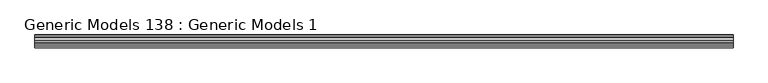
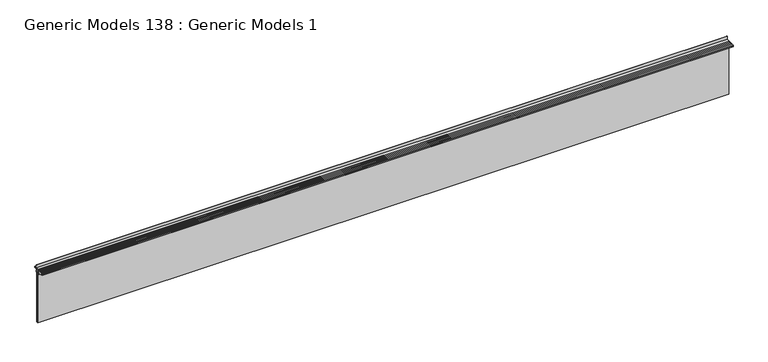
"""IFC4 building model written with IfcOpenShell, lengths in millimetres: proxy geometry, Generic Models 138 : Generic Models 1."""

from ifc_helpers import new_model, si_unit, point, frame, frame_2d, origin, place, context, project, spatial, polyline, circle_curve, trimmed, segment, composite_curve, outline, extrude, source, transform, mapped, element, save


def generic_models_138_generic_models_1_f7e5df14(model_context):
    return source(origin(), model_context, "Body", "SweptSolid", [
        extrude(outline(composite_curve([segment(polyline([(11384.4166338, 129382.901), (11402.4851772, 129382.901), (11402.4851772, 129379.726), (11404.7711811, 129379.726), (11404.7711811, 129382.901), (11422.2789303, 129382.901), (11422.2789303, 129379.726), (11424.5649341, 129379.726), (11424.5649341, 129382.901), (11441.5920338, 129382.901), (11441.5920338, 129380.8182), (11444.7670338, 129380.8182), (11444.7670338, 129382.901), (11461.8664163, 129382.901), (11461.8664163, 129379.726), (11464.1524163, 129379.726), (11464.1524163, 129382.901), (11500.6215842, 129382.901), (11500.6215842, 129418.2728876)]), True, "CONTINUOUS"), segment(trimmed(circle_curve(frame_2d((11501.3200844, 129418.2705467)), 0.6985041), [point((11500.6215842, 129418.2728876))], [point((11502.0185842, 129418.268087))], False, "CARTESIAN"), True, "CONTINUOUS"), segment(polyline([(11502.0185842, 129418.268087), (11502.0185842, 129382.901), (11526.9064186, 129382.901), (11526.9064186, 129381.504), (11520.5564186, 129381.504), (11520.5564186, 129379.218), (11528.4599842, 129379.218), (11528.4599842, 129370.2865766), (11500.5961842, 129367.8642068), (11465.6457842, 129367.8642068), (11465.6457842, 129362.9874141), (11461.632657, 129362.9874141), (11461.632657, 129369.4063537), (11459.6513826, 129369.4063537), (11459.6513826, 129361.4561607), (11451.2440469, 129361.4561607), (11451.2440469, 129360.5163642), (11433.7180469, 129360.5163642), (11433.7180469, 129358.2303642), (11451.2440469, 129358.2303642), (11451.2440469, 129349.5435642), (11454.2920198, 129349.5435642), (11454.2920198, 129346.3685642), (11424.8787958, 129346.3685642), (11424.8787958, 129352.7003967), (11405.8287958, 129352.7003967), (11405.8287958, 129355.0879932), (11404.2286028, 129355.0879932), (11400.2916338, 129358.2629932), (11398.6914407, 129358.2629932), (11398.6914407, 129362.2253967), (11395.5164407, 129362.2253967), (11394.7289888, 129363.0381862), (11384.4166338, 129363.0381862), (11384.4166338, 129372.9696052), (11392.3668268, 129372.9696052), (11392.3668268, 129374.9507827), (11384.4166338, 129374.9507827), (11384.4166338, 129382.901)]), True, "CONTINUOUS")], self_intersect=False)), frame((-5398.5537428, 0.0, 0.0), z_axis=(1.0, 0.0, 0.0), x_axis=(0.0, 1.0, 0.0)), (0.0, 0.0, 1.0), 7886.7),
        extrude(outline(composite_curve([segment(polyline([(11492.1197262, 129334.0440891), (11491.0965842, 129335.0672312), (11491.0965842, 129338.64785), (11469.6592133, 129338.64785), (11472.0475021, 129336.2595612), (11472.0475021, 129326.3281612), (11460.2198217, 129327.3408112), (11460.2198217, 129329.5031612), (11456.4519021, 129329.5031612), (11456.4519021, 129337.0469612), (11458.0521021, 129337.0469612), (11458.0521021, 129338.64785), (11456.1715842, 129338.64785), (11456.1715842, 129356.93585)]), True, "CONTINUOUS"), segment(trimmed(circle_curve(frame_2d((11456.9843842, 129356.93585)), 0.8128), [point((11456.1715842, 129356.93585))], [point((11456.9843842, 129357.74865))], False, "CARTESIAN"), True, "CONTINUOUS"), segment(polyline([(11456.9843842, 129357.74865), (11470.3193842, 129357.74865)]), True, "CONTINUOUS"), segment(trimmed(circle_curve(frame_2d((11472.3005842, 129357.74865)), 1.9812), [point((11470.3193842, 129357.74865))], [point((11474.2817842, 129357.74865))], True, "CARTESIAN"), True, "CONTINUOUS"), segment(polyline([(11474.2817842, 129357.74865), (11486.4737842, 129357.74865), (11486.4737842, 129363.05725), (11492.0871842, 129363.05725), (11492.0871842, 129355.13245), (11493.9921842, 129355.13245), (11493.9921842, 129358.43445), (11495.6685842, 129358.43445), (11495.6685842, 129360.46645), (11498.2339842, 129360.46645)]), True, "CONTINUOUS"), segment(trimmed(circle_curve(frame_2d((11498.2339842, 129358.07885)), 2.3876), [point((11498.2339842, 129360.46645))], [point((11500.6215842, 129358.07885))], False, "CARTESIAN"), True, "CONTINUOUS"), segment(polyline([(11500.6215842, 129358.07885), (11500.6215842, 129335.77765), (11498.2339842, 129335.77765), (11495.6986236, 129327.9718265), (11493.2555842, 129327.7822761), (11493.2555842, 129329.80865), (11492.1197262, 129329.80865), (11492.1197262, 129334.0440891)]), True, "CONTINUOUS")], self_intersect=False)), frame((-5398.5537428, 0.0, 0.0), z_axis=(1.0, 0.0, 0.0), x_axis=(0.0, 1.0, 0.0)), (0.0, 0.0, 1.0), 7886.7),
        extrude(outline(polyline([(-5398.5537428, 11472.8412521), (-5398.5537428, 11477.6037521), (2488.1462572, 11477.6037521), (2488.1462572, 11472.8412521), (-5398.5537428, 11472.8412521)])), frame((0.0, 0.0, 128735.5165519), z_axis=(0.0, 0.0, 1.0), x_axis=(1.0, 0.0, 0.0)), (0.0, 0.0, 1.0), 602.3375481),
        extrude(outline(polyline([(-5398.5537428, 11478.3975021), (-5398.5537428, 11484.7465842), (2488.1462572, 11484.7465842), (2488.1462572, 11478.3975021), (-5398.5537428, 11478.3975021)])), frame((0.0, 0.0, 129331.5041), z_axis=(0.0, 0.0, 1.0), x_axis=(1.0, 0.0, 0.0)), (0.0, 0.0, 1.0), 6.35),
        extrude(outline(polyline([(-5398.5537428, 11485.5403342), (-5398.5537428, 11490.3028342), (2488.1462572, 11490.3028342), (2488.1462572, 11485.5403342), (-5398.5537428, 11485.5403342)])), frame((0.0, 0.0, 128735.5165519), z_axis=(0.0, 0.0, 1.0), x_axis=(1.0, 0.0, 0.0)), (0.0, 0.0, 1.0), 602.3375481),
    ])


if __name__ == "__main__":
    model = new_model("IFC4")
    model_context = context("Model", 3, world=origin())
    ifc_project = project(units=[si_unit("LENGTHUNIT", "METRE", prefix="MILLI")], contexts=[model_context])
    site = spatial("IfcSite", under=ifc_project)
    building = spatial("IfcBuilding", under=site)
    placement = place(None, origin())
    generic_models_138_generic_models_1_shape = generic_models_138_generic_models_1_f7e5df14(model_context)
    element("IfcBuildingElementProxy", 1, Name="Generic Models 138 : Generic Models 1", ObjectType="Generic Models 138 : Generic Models 1", at=placement, inside=building, context=model_context, shape_type="MappedRepresentation", body=[
        mapped(generic_models_138_generic_models_1_shape, transform((0.0, 0.0, 0.0), x_axis=(1.0, 0.0, 0.0), y_axis=(0.0, 1.0, 0.0), z_axis=(0.0, 0.0, 1.0))),
    ])
    save(model, "model.ifc")

# Revit data of these elements
# Element 1 (IfcBuildingElementProxy, "Generic Models 138 : Generic Models 1")
#   Materials on its faces: "_WINDOW PER SCHEDULE"
# Materials
#   "_WINDOW PER SCHEDULE": class "Generic", colour RGB 255 255 255, transparency 0, Cost = 0
